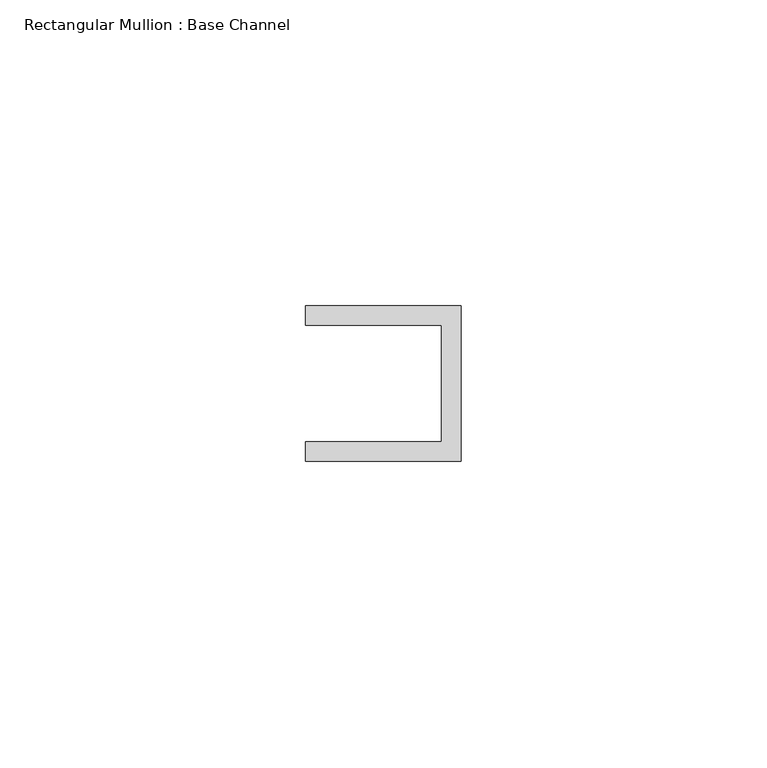
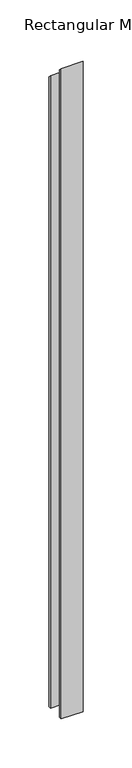
"""IFC4 building model written with IfcOpenShell, lengths in millimetres: member geometry, Rectangular Mullion : Base Channel."""

from ifc_helpers import new_model, si_unit, origin, place, context, project, spatial, faceted_brep, source, transform, mapped, element, save


def rectangular_mullion_base_channel_f13e1730(model_context):
    return source(origin(), model_context, "Body", "Brep", [
        faceted_brep([(0.0, -12.7, -797.4591001), (-25.4, -12.7, -797.4591001), (-25.4, -9.525, -797.4591001), (-3.175, -9.525, -797.4591001), (-3.175, 9.525, -797.4591001), (-25.4, 9.525, -797.4591001), (-25.4, 12.7, -797.4591001), (0.0, 12.7, -797.4591001), (0.0, 12.7, -12.7), (0.0, -12.7, 12.7), (-25.4, 12.7, -12.7), (-25.4, 9.525, -9.525), (-3.175, 9.525, -9.525), (-3.175, -9.525, 9.525), (-25.4, -9.525, 9.525), (-25.4, -12.7, 12.7)], [[[0, 1, 2, 3, 4, 5, 6, 7]], [[8, 9, 0, 7]], [[10, 8, 7, 6]], [[11, 10, 6, 5]], [[12, 11, 5, 4]], [[13, 12, 4, 3]], [[14, 13, 3, 2]], [[15, 14, 2, 1]], [[9, 15, 1, 0]], [[9, 8, 10, 11, 12, 13, 14, 15]]]),
    ])


if __name__ == "__main__":
    model = new_model("IFC4")
    model_context = context("Model", 3, world=origin())
    ifc_project = project(units=[si_unit("LENGTHUNIT", "METRE", prefix="MILLI")], contexts=[model_context])
    site = spatial("IfcSite", under=ifc_project)
    building = spatial("IfcBuilding", under=site)
    placement = place(None, origin())
    rectangular_mullion_base_channel_shape = rectangular_mullion_base_channel_f13e1730(model_context)
    element("IfcMember", 1, ObjectType="Rectangular Mullion : Base Channel", at=placement, inside=building, context=model_context, shape_type="MappedRepresentation", body=[
        mapped(rectangular_mullion_base_channel_shape, transform((0.0, 0.0, 0.0), x_axis=(1.0, 0.0, 0.0), y_axis=(0.0, 1.0, 0.0), z_axis=(0.0, 0.0, 1.0))),
    ])
    save(model, "model.ifc")

# Revit data of these elements
# Type "Rectangular Mullion : Base Channel"
#   built-in parameter 1007322 = 0.0833333 (stored number, unit not read)
#   built-in parameter 1007321 = 0.0416667 (stored number, unit not read)
#   built-in parameter 1007320 = -0.03125 (stored number, unit not read)
# Element 1 (IfcMember, "Rectangular Mullion : Base Channel")
#   Materials on its faces: "ALUM"
# Materials
#   "ALUM": class "Generic", colour RGB 157 157 157, transparency 0, Cost = 0
